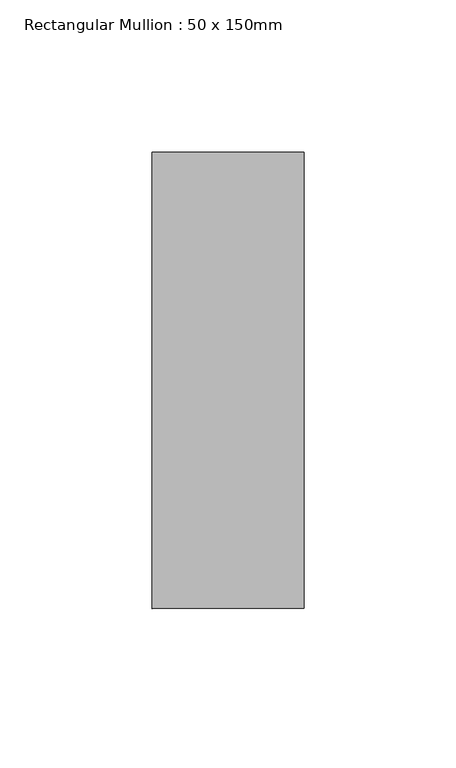
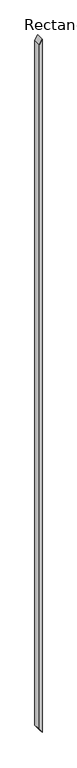
"""IFC4 building model written with IfcOpenShell, lengths in millimetres: member geometry, Rectangular Mullion : 50 x 150mm."""

from ifc_helpers import new_model, si_unit, frame, origin, place, context, project, spatial, polyline, outline, extrude, source, transform, mapped, element, save


def rectangular_mullion_50_x_150mm_e862281f(model_context):
    return source(origin(), model_context, "Body", "SweptSolid", [
        extrude(outline(polyline([(0.0, 0.0), (-85.321119, -50.0), (-13880.4605319, -50.0), (-13952.0824058, 0.0), (0.0, 0.0)])), frame((0.0, -75.0, 0.0), z_axis=(0.0, 1.0, 0.0), x_axis=(0.0, 0.0, 1.0)), (0.0, 0.0, 1.0), 150.0),
    ])


if __name__ == "__main__":
    model = new_model("IFC4")
    model_context = context("Model", 3, world=origin())
    ifc_project = project(units=[si_unit("LENGTHUNIT", "METRE", prefix="MILLI")], contexts=[model_context])
    site = spatial("IfcSite", under=ifc_project)
    building = spatial("IfcBuilding", under=site)
    placement = place(None, origin())
    rectangular_mullion_50_x_150mm_shape = rectangular_mullion_50_x_150mm_e862281f(model_context)
    element("IfcMember", 1, ObjectType="Rectangular Mullion : 50 x 150mm", at=placement, inside=building, context=model_context, shape_type="MappedRepresentation", body=[
        mapped(rectangular_mullion_50_x_150mm_shape, transform((0.0, 0.0, 0.0), x_axis=(1.0, 0.0, 0.0), y_axis=(0.0, 1.0, 0.0), z_axis=(0.0, 0.0, 1.0))),
    ])
    save(model, "model.ifc")

# Revit data of these elements
# Type "Rectangular Mullion : 50 x 150mm"
#   built-in parameter 1007304 = 0.492126 (stored number, unit not read)
#   built-in parameter 1007301 = 0.082021 (stored number, unit not read)
#   built-in parameter 1007300 = 0.082021 (stored number, unit not read)
# Element 1 (IfcMember, "Rectangular Mullion : 50 x 150mm")
#   Materials on its faces: "Metal - Aluminium"
# Materials
#   "Metal - Aluminium": class "Metal", colour RGB 247 247 247, transparency 0
